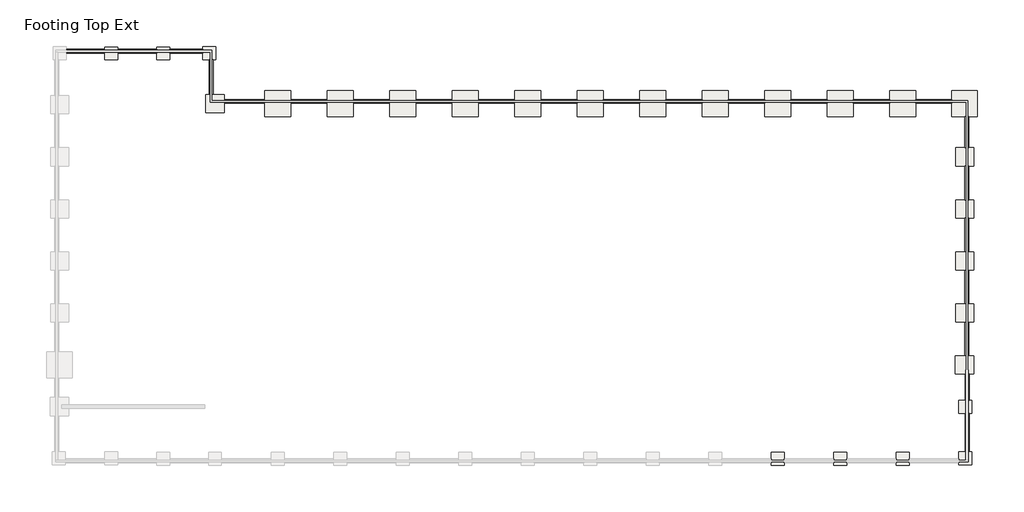
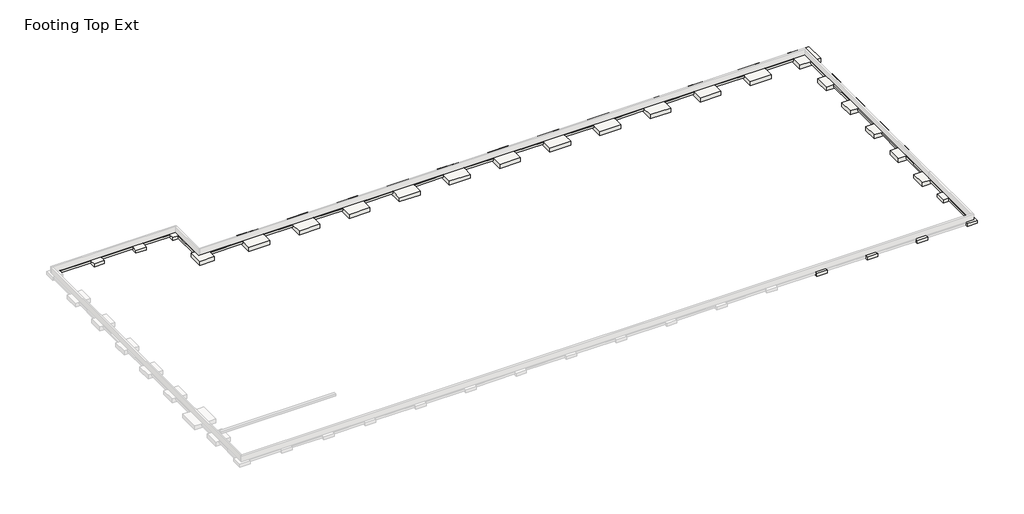
# One storey, part 2 of 2: 26 slabs, 5 footings.
"""IFC4 building model written with IfcOpenShell, lengths in millimetres."""

from ifc_helpers import new_model, si_unit, frame, origin, place, context, project, spatial, polyline, outline, extrude, faceted_brep, element, save

model = new_model("IFC4")

# Units and contexts
model_context = context("Model", 3, world=origin())
ifc_project = project(units=[si_unit("LENGTHUNIT", "METRE", prefix="MILLI")], contexts=[model_context])

# Site, building, storey
site = spatial("IfcSite", under=ifc_project)
building = spatial("IfcBuilding", under=site)
storey = spatial("IfcBuildingStorey", under=building, Name="Footing Top Ext", Elevation=-914.4)

# Footings
placement = place(None, origin())
element("IfcFooting", 1, ObjectType="Bearing Footing - 18\" x 12\"", at=placement, inside=storey, context=model_context, shape_type="SweptSolid", body=[
    extrude(outline(polyline([(305697.0398264, -530975.6413841), (305697.0398264, -530518.4413841), (310230.9398264, -530518.4413841), (310230.9398264, -530975.6413841), (305697.0398264, -530975.6413841)])), frame((0.0, 0.0, -1219.2), z_axis=(0.0, 0.0, 1.0), x_axis=(1.0, 0.0, 0.0)), (0.0, 0.0, 1.0), 304.8),
    extrude(outline(polyline([(317882.6898264, -530975.6413841), (317882.6898264, -530518.4413841), (321806.9898264, -530518.4413841), (321806.9898264, -530975.6413841), (317882.6898264, -530975.6413841)])), frame((0.0, 0.0, -1219.2), z_axis=(0.0, 0.0, 1.0), x_axis=(1.0, 0.0, 0.0)), (0.0, 0.0, 1.0), 304.8),
    extrude(outline(polyline([(316358.6898264, -530518.4413841), (316358.6898264, -530975.6413841), (311754.9398264, -530975.6413841), (311754.9398264, -530518.4413841), (316358.6898264, -530518.4413841)])), frame((0.0, 0.0, -1219.2), z_axis=(0.0, 0.0, 1.0), x_axis=(1.0, 0.0, 0.0)), (0.0, 0.0, 1.0), 304.8),
])
element("IfcFooting", 2, ObjectType="Bearing Footing - 18\" x 12\"", at=placement, inside=storey, context=model_context, shape_type="SweptSolid", body=[
    extrude(outline(polyline([(322537.2398264, -531712.2413841), (322994.4398264, -531712.2413841), (322994.4398264, -535839.7413841), (322537.2398264, -535839.7413841), (322537.2398264, -531712.2413841)])), frame((0.0, 0.0, -1219.2), z_axis=(0.0, 0.0, 1.0), x_axis=(1.0, 0.0, 0.0)), (0.0, 0.0, 1.0), 304.8),
])
element("IfcFooting", 3, ObjectType="Bearing Footing - 18\" x 12\"", at=placement, inside=storey, context=model_context, shape_type="SweptSolid", body=[
    extrude(outline(polyline([(409862.4397781, -536430.2913841), (409862.4397781, -536887.4913841), (405658.7398264, -536887.4913841), (405658.7398264, -536430.2913841), (409862.4397781, -536430.2913841)])), frame((0.0, 0.0, -1219.2), z_axis=(0.0, 0.0, 1.0), x_axis=(1.0, 0.0, 0.0)), (0.0, 0.0, 1.0), 304.8),
    extrude(outline(polyline([(402610.7398264, -536430.2913841), (402610.7398264, -536887.4913841), (398305.4398264, -536887.4913841), (398305.4398264, -536430.2913841), (402610.7398264, -536430.2913841)])), frame((0.0, 0.0, -1219.2), z_axis=(0.0, 0.0, 1.0), x_axis=(1.0, 0.0, 0.0)), (0.0, 0.0, 1.0), 304.8),
    extrude(outline(polyline([(395257.4398264, -536430.2913841), (395257.4398264, -536887.4913841), (390952.1398264, -536887.4913841), (390952.1398264, -536430.2913841), (395257.4398264, -536430.2913841)])), frame((0.0, 0.0, -1219.2), z_axis=(0.0, 0.0, 1.0), x_axis=(1.0, 0.0, 0.0)), (0.0, 0.0, 1.0), 304.8),
    extrude(outline(polyline([(387904.1398264, -536430.2913841), (387904.1398264, -536887.4913841), (383598.8398264, -536887.4913841), (383598.8398264, -536430.2913841), (387904.1398264, -536430.2913841)])), frame((0.0, 0.0, -1219.2), z_axis=(0.0, 0.0, 1.0), x_axis=(1.0, 0.0, 0.0)), (0.0, 0.0, 1.0), 304.8),
    extrude(outline(polyline([(380550.8398264, -536430.2913841), (380550.8398264, -536887.4913841), (376245.5398264, -536887.4913841), (376245.5398264, -536430.2913841), (380550.8398264, -536430.2913841)])), frame((0.0, 0.0, -1219.2), z_axis=(0.0, 0.0, 1.0), x_axis=(1.0, 0.0, 0.0)), (0.0, 0.0, 1.0), 304.8),
    extrude(outline(polyline([(373197.5398264, -536430.2913841), (373197.5398264, -536887.4913841), (368892.2398264, -536887.4913841), (368892.2398264, -536430.2913841), (373197.5398264, -536430.2913841)])), frame((0.0, 0.0, -1219.2), z_axis=(0.0, 0.0, 1.0), x_axis=(1.0, 0.0, 0.0)), (0.0, 0.0, 1.0), 304.8),
    extrude(outline(polyline([(365844.2398264, -536430.2913841), (365844.2398264, -536887.4913841), (361538.9398264, -536887.4913841), (361538.9398264, -536430.2913841), (365844.2398264, -536430.2913841)])), frame((0.0, 0.0, -1219.2), z_axis=(0.0, 0.0, 1.0), x_axis=(1.0, 0.0, 0.0)), (0.0, 0.0, 1.0), 304.8),
    extrude(outline(polyline([(358490.9398264, -536430.2913841), (358490.9398264, -536887.4913841), (354185.6398264, -536887.4913841), (354185.6398264, -536430.2913841), (358490.9398264, -536430.2913841)])), frame((0.0, 0.0, -1219.2), z_axis=(0.0, 0.0, 1.0), x_axis=(1.0, 0.0, 0.0)), (0.0, 0.0, 1.0), 304.8),
    extrude(outline(polyline([(351137.6398264, -536430.2913841), (351137.6398264, -536887.4913841), (346832.3398264, -536887.4913841), (346832.3398264, -536430.2913841), (351137.6398264, -536430.2913841)])), frame((0.0, 0.0, -1219.2), z_axis=(0.0, 0.0, 1.0), x_axis=(1.0, 0.0, 0.0)), (0.0, 0.0, 1.0), 304.8),
    extrude(outline(polyline([(343784.3398264, -536430.2913841), (343784.3398264, -536887.4913841), (339479.0398264, -536887.4913841), (339479.0398264, -536430.2913841), (343784.3398264, -536430.2913841)])), frame((0.0, 0.0, -1219.2), z_axis=(0.0, 0.0, 1.0), x_axis=(1.0, 0.0, 0.0)), (0.0, 0.0, 1.0), 304.8),
    extrude(outline(polyline([(336431.0398264, -536430.2913841), (336431.0398264, -536887.4913841), (332125.7398264, -536887.4913841), (332125.7398264, -536430.2913841), (336431.0398264, -536430.2913841)])), frame((0.0, 0.0, -1219.2), z_axis=(0.0, 0.0, 1.0), x_axis=(1.0, 0.0, 0.0)), (0.0, 0.0, 1.0), 304.8),
    extrude(outline(polyline([(329077.7398264, -536430.2913841), (329077.7398264, -536887.4913841), (324289.8398264, -536887.4913841), (324289.8398264, -536430.2913841), (329077.7398264, -536430.2913841)])), frame((0.0, 0.0, -1219.2), z_axis=(0.0, 0.0, 1.0), x_axis=(1.0, 0.0, 0.0)), (0.0, 0.0, 1.0), 304.8),
])
element("IfcFooting", 4, ObjectType="Bearing Footing - 18\" x 12\"", at=placement, inside=storey, context=model_context, shape_type="SweptSolid", body=[
    extrude(outline(polyline([(411894.4398264, -560496.7913841), (411437.2398264, -560496.7913841), (411437.2398264, -556502.6413841), (411894.4398264, -556502.6413841), (411894.4398264, -560496.7913841)])), frame((0.0, 0.0, -1219.2), z_axis=(0.0, 0.0, 1.0), x_axis=(1.0, 0.0, 0.0)), (0.0, 0.0, 1.0), 304.8),
    extrude(outline(polyline([(411437.2398264, -562630.3913841), (411894.4398264, -562630.3913841), (411894.4398264, -566599.1414082), (411437.2398264, -566599.1414082), (411437.2398264, -562630.3913841)])), frame((0.0, 0.0, -1219.2), z_axis=(0.0, 0.0, 1.0), x_axis=(1.0, 0.0, 0.0)), (0.0, 0.0, 1.0), 304.8),
    extrude(outline(polyline([(411894.4398264, -554369.0413841), (411437.2398264, -554369.0413841), (411437.2398264, -550374.8913841), (411894.4398264, -550374.8913841), (411894.4398264, -554369.0413841)])), frame((0.0, 0.0, -1219.2), z_axis=(0.0, 0.0, 1.0), x_axis=(1.0, 0.0, 0.0)), (0.0, 0.0, 1.0), 304.8),
    extrude(outline(polyline([(411894.4398264, -548241.2913841), (411437.2398264, -548241.2913841), (411437.2398264, -544247.1413841), (411894.4398264, -544247.1413841), (411894.4398264, -548241.2913841)])), frame((0.0, 0.0, -1219.2), z_axis=(0.0, 0.0, 1.0), x_axis=(1.0, 0.0, 0.0)), (0.0, 0.0, 1.0), 304.8),
    extrude(outline(polyline([(411894.4398264, -542113.5413841), (411437.2398264, -542113.5413841), (411437.2398264, -538424.1913358), (411894.4398264, -538424.1913358), (411894.4398264, -542113.5413841)])), frame((0.0, 0.0, -1219.2), z_axis=(0.0, 0.0, 1.0), x_axis=(1.0, 0.0, 0.0)), (0.0, 0.0, 1.0), 304.8),
])
element("IfcFooting", 5, ObjectType="Bearing Footing - 18\" x 12\"", at=placement, inside=storey, context=model_context, shape_type="SweptSolid", body=[
    extrude(outline(polyline([(411932.5398264, -571831.5413841), (411475.3398264, -571831.5413841), (411475.3398264, -568732.7414082), (411932.5398264, -568732.7414082), (411932.5398264, -571831.5413841)])), frame((0.0, 0.0, -1219.2), z_axis=(0.0, 0.0, 1.0), x_axis=(1.0, 0.0, 0.0)), (0.0, 0.0, 1.0), 304.8),
    extrude(outline(polyline([(411475.3398264, -573355.5413841), (411932.5398264, -573355.5413841), (411932.5398264, -577927.5413841), (411475.3398264, -577927.5413841), (411475.3398264, -573355.5413841)])), frame((0.0, 0.0, -1219.2), z_axis=(0.0, 0.0, 1.0), x_axis=(1.0, 0.0, 0.0)), (0.0, 0.0, 1.0), 304.8),
])

# Slabs
element("IfcSlab", 6, ObjectType="Footing-Rectangular : F10", at=placement, inside=storey, context=model_context, shape_type="Brep", body=[
    faceted_brep([(409862.4397781, -535376.1913358, -914.4), (409862.4397781, -536430.2913841, -914.4), (409862.4397781, -536887.4913841, -914.4), (409862.4397781, -538424.1913358, -914.4), (411437.2398264, -538424.1913358, -914.4), (411894.4398264, -538424.1913358, -914.4), (412910.4397781, -538424.1913358, -914.4), (412910.4397781, -535376.1913358, -914.4), (409862.4397781, -535376.1913358, -1524.0), (412910.4397781, -535376.1913358, -1524.0), (412910.4397781, -538424.1913358, -1524.0), (409862.4397781, -538424.1913358, -1524.0)], [[[0, 1, 2, 3, 4, 5, 6, 7]], [[8, 9, 10, 11]], [[3, 2, 1, 0, 8, 11]], [[6, 5, 4, 3, 11, 10]], [[7, 6, 10, 9]], [[0, 7, 9, 8]]]),
])
element("IfcSlab", 7, ObjectType="Footing-Rectangular : F10", at=placement, inside=storey, context=model_context, shape_type="Brep", body=[
    faceted_brep([(402610.7398264, -535382.5413358, -914.4), (402610.7398264, -536430.2913841, -914.4), (402610.7398264, -536887.4913841, -914.4), (402610.7398264, -538430.5413358, -914.4), (405658.7398264, -538430.5413358, -914.4), (405658.7398264, -536887.4913841, -914.4), (405658.7398264, -536430.2913841, -914.4), (405658.7398264, -535382.5413358, -914.4), (402610.7398264, -535382.5413358, -1524.0), (405658.7398264, -535382.5413358, -1524.0), (405658.7398264, -538430.5413358, -1524.0), (402610.7398264, -538430.5413358, -1524.0)], [[[0, 1, 2, 3, 4, 5, 6, 7]], [[8, 9, 10, 11]], [[3, 2, 1, 0, 8, 11]], [[4, 3, 11, 10]], [[7, 6, 5, 4, 10, 9]], [[0, 7, 9, 8]]]),
])
element("IfcSlab", 8, ObjectType="Footing-Rectangular : F10", at=placement, inside=storey, context=model_context, shape_type="Brep", body=[
    faceted_brep([(395257.4398264, -535382.5413358, -914.4), (395257.4398264, -536430.2913841, -914.4), (395257.4398264, -536887.4913841, -914.4), (395257.4398264, -538430.5413358, -914.4), (398305.4398264, -538430.5413358, -914.4), (398305.4398264, -536887.4913841, -914.4), (398305.4398264, -536430.2913841, -914.4), (398305.4398264, -535382.5413358, -914.4), (395257.4398264, -535382.5413358, -1524.0), (398305.4398264, -535382.5413358, -1524.0), (398305.4398264, -538430.5413358, -1524.0), (395257.4398264, -538430.5413358, -1524.0)], [[[0, 1, 2, 3, 4, 5, 6, 7]], [[8, 9, 10, 11]], [[3, 2, 1, 0, 8, 11]], [[4, 3, 11, 10]], [[7, 6, 5, 4, 10, 9]], [[0, 7, 9, 8]]]),
])
element("IfcSlab", 9, ObjectType="Footing-Rectangular : F10", at=placement, inside=storey, context=model_context, shape_type="Brep", body=[
    faceted_brep([(387904.1398264, -535382.5413358, -914.4), (387904.1398264, -536430.2913841, -914.4), (387904.1398264, -536887.4913841, -914.4), (387904.1398264, -538430.5413358, -914.4), (390952.1398264, -538430.5413358, -914.4), (390952.1398264, -536887.4913841, -914.4), (390952.1398264, -536430.2913841, -914.4), (390952.1398264, -535382.5413358, -914.4), (387904.1398264, -535382.5413358, -1524.0), (390952.1398264, -535382.5413358, -1524.0), (390952.1398264, -538430.5413358, -1524.0), (387904.1398264, -538430.5413358, -1524.0)], [[[0, 1, 2, 3, 4, 5, 6, 7]], [[8, 9, 10, 11]], [[3, 2, 1, 0, 8, 11]], [[4, 3, 11, 10]], [[7, 6, 5, 4, 10, 9]], [[0, 7, 9, 8]]]),
])
element("IfcSlab", 10, ObjectType="Footing-Rectangular : F10", at=placement, inside=storey, context=model_context, shape_type="Brep", body=[
    faceted_brep([(380550.8398264, -535382.5413358, -914.4), (380550.8398264, -536430.2913841, -914.4), (380550.8398264, -536887.4913841, -914.4), (380550.8398264, -538430.5413358, -914.4), (383598.8398264, -538430.5413358, -914.4), (383598.8398264, -536887.4913841, -914.4), (383598.8398264, -536430.2913841, -914.4), (383598.8398264, -535382.5413358, -914.4), (380550.8398264, -535382.5413358, -1524.0), (383598.8398264, -535382.5413358, -1524.0), (383598.8398264, -538430.5413358, -1524.0), (380550.8398264, -538430.5413358, -1524.0)], [[[0, 1, 2, 3, 4, 5, 6, 7]], [[8, 9, 10, 11]], [[3, 2, 1, 0, 8, 11]], [[4, 3, 11, 10]], [[7, 6, 5, 4, 10, 9]], [[0, 7, 9, 8]]]),
])
element("IfcSlab", 11, ObjectType="Footing-Rectangular : F10", at=placement, inside=storey, context=model_context, shape_type="Brep", body=[
    faceted_brep([(373197.5398264, -535382.5413358, -914.4), (373197.5398264, -536430.2913841, -914.4), (373197.5398264, -536887.4913841, -914.4), (373197.5398264, -538430.5413358, -914.4), (376245.5398264, -538430.5413358, -914.4), (376245.5398264, -536887.4913841, -914.4), (376245.5398264, -536430.2913841, -914.4), (376245.5398264, -535382.5413358, -914.4), (373197.5398264, -535382.5413358, -1524.0), (376245.5398264, -535382.5413358, -1524.0), (376245.5398264, -538430.5413358, -1524.0), (373197.5398264, -538430.5413358, -1524.0)], [[[0, 1, 2, 3, 4, 5, 6, 7]], [[8, 9, 10, 11]], [[3, 2, 1, 0, 8, 11]], [[4, 3, 11, 10]], [[7, 6, 5, 4, 10, 9]], [[0, 7, 9, 8]]]),
])
element("IfcSlab", 12, ObjectType="Footing-Rectangular : F10", at=placement, inside=storey, context=model_context, shape_type="Brep", body=[
    faceted_brep([(365844.2398264, -535382.5413358, -914.4), (365844.2398264, -536430.2913841, -914.4), (365844.2398264, -536887.4913841, -914.4), (365844.2398264, -538430.5413358, -914.4), (368892.2398264, -538430.5413358, -914.4), (368892.2398264, -536887.4913841, -914.4), (368892.2398264, -536430.2913841, -914.4), (368892.2398264, -535382.5413358, -914.4), (365844.2398264, -535382.5413358, -1524.0), (368892.2398264, -535382.5413358, -1524.0), (368892.2398264, -538430.5413358, -1524.0), (365844.2398264, -538430.5413358, -1524.0)], [[[0, 1, 2, 3, 4, 5, 6, 7]], [[8, 9, 10, 11]], [[3, 2, 1, 0, 8, 11]], [[4, 3, 11, 10]], [[7, 6, 5, 4, 10, 9]], [[0, 7, 9, 8]]]),
])
element("IfcSlab", 13, ObjectType="Footing-Rectangular : F10", at=placement, inside=storey, context=model_context, shape_type="Brep", body=[
    faceted_brep([(358490.9398264, -535382.5413358, -914.4), (358490.9398264, -536430.2913841, -914.4), (358490.9398264, -536887.4913841, -914.4), (358490.9398264, -538430.5413358, -914.4), (361538.9398264, -538430.5413358, -914.4), (361538.9398264, -536887.4913841, -914.4), (361538.9398264, -536430.2913841, -914.4), (361538.9398264, -535382.5413358, -914.4), (358490.9398264, -535382.5413358, -1524.0), (361538.9398264, -535382.5413358, -1524.0), (361538.9398264, -538430.5413358, -1524.0), (358490.9398264, -538430.5413358, -1524.0)], [[[0, 1, 2, 3, 4, 5, 6, 7]], [[8, 9, 10, 11]], [[3, 2, 1, 0, 8, 11]], [[4, 3, 11, 10]], [[7, 6, 5, 4, 10, 9]], [[0, 7, 9, 8]]]),
])
element("IfcSlab", 14, ObjectType="Footing-Rectangular : F10", at=placement, inside=storey, context=model_context, shape_type="Brep", body=[
    faceted_brep([(351137.6398264, -535382.5413358, -914.4), (351137.6398264, -536430.2913841, -914.4), (351137.6398264, -536887.4913841, -914.4), (351137.6398264, -538430.5413358, -914.4), (354185.6398264, -538430.5413358, -914.4), (354185.6398264, -536887.4913841, -914.4), (354185.6398264, -536430.2913841, -914.4), (354185.6398264, -535382.5413358, -914.4), (351137.6398264, -535382.5413358, -1524.0), (354185.6398264, -535382.5413358, -1524.0), (354185.6398264, -538430.5413358, -1524.0), (351137.6398264, -538430.5413358, -1524.0)], [[[0, 1, 2, 3, 4, 5, 6, 7]], [[8, 9, 10, 11]], [[3, 2, 1, 0, 8, 11]], [[4, 3, 11, 10]], [[7, 6, 5, 4, 10, 9]], [[0, 7, 9, 8]]]),
])
element("IfcSlab", 15, ObjectType="Footing-Rectangular : F10", at=placement, inside=storey, context=model_context, shape_type="Brep", body=[
    faceted_brep([(343784.3398264, -535382.5413358, -914.4), (343784.3398264, -536430.2913841, -914.4), (343784.3398264, -536887.4913841, -914.4), (343784.3398264, -538430.5413358, -914.4), (346832.3398264, -538430.5413358, -914.4), (346832.3398264, -536887.4913841, -914.4), (346832.3398264, -536430.2913841, -914.4), (346832.3398264, -535382.5413358, -914.4), (343784.3398264, -535382.5413358, -1524.0), (346832.3398264, -535382.5413358, -1524.0), (346832.3398264, -538430.5413358, -1524.0), (343784.3398264, -538430.5413358, -1524.0)], [[[0, 1, 2, 3, 4, 5, 6, 7]], [[8, 9, 10, 11]], [[3, 2, 1, 0, 8, 11]], [[4, 3, 11, 10]], [[7, 6, 5, 4, 10, 9]], [[0, 7, 9, 8]]]),
])
element("IfcSlab", 16, ObjectType="Footing-Rectangular : F10", at=placement, inside=storey, context=model_context, shape_type="Brep", body=[
    faceted_brep([(336431.0398264, -535382.5413358, -914.4), (336431.0398264, -536430.2913841, -914.4), (336431.0398264, -536887.4913841, -914.4), (336431.0398264, -538430.5413358, -914.4), (339479.0398264, -538430.5413358, -914.4), (339479.0398264, -536887.4913841, -914.4), (339479.0398264, -536430.2913841, -914.4), (339479.0398264, -535382.5413358, -914.4), (336431.0398264, -535382.5413358, -1524.0), (339479.0398264, -535382.5413358, -1524.0), (339479.0398264, -538430.5413358, -1524.0), (336431.0398264, -538430.5413358, -1524.0)], [[[0, 1, 2, 3, 4, 5, 6, 7]], [[8, 9, 10, 11]], [[3, 2, 1, 0, 8, 11]], [[4, 3, 11, 10]], [[7, 6, 5, 4, 10, 9]], [[0, 7, 9, 8]]]),
])
element("IfcSlab", 17, ObjectType="Footing-Rectangular : F10", at=placement, inside=storey, context=model_context, shape_type="Brep", body=[
    faceted_brep([(329077.7398264, -535382.5413358, -914.4), (329077.7398264, -536430.2913841, -914.4), (329077.7398264, -536887.4913841, -914.4), (329077.7398264, -538430.5413358, -914.4), (332125.7398264, -538430.5413358, -914.4), (332125.7398264, -536887.4913841, -914.4), (332125.7398264, -536430.2913841, -914.4), (332125.7398264, -535382.5413358, -914.4), (329077.7398264, -535382.5413358, -1524.0), (332125.7398264, -535382.5413358, -1524.0), (332125.7398264, -538430.5413358, -1524.0), (329077.7398264, -538430.5413358, -1524.0)], [[[0, 1, 2, 3, 4, 5, 6, 7]], [[8, 9, 10, 11]], [[3, 2, 1, 0, 8, 11]], [[4, 3, 11, 10]], [[7, 6, 5, 4, 10, 9]], [[0, 7, 9, 8]]]),
])
element("IfcSlab", 18, ObjectType="Footing-Rectangular : F5", at=placement, inside=storey, context=model_context, shape_type="Brep", body=[
    faceted_brep([(317882.6898264, -530245.3913841, -914.4), (316358.6898264, -530245.3913841, -914.4), (316358.6898264, -530518.4413841, -914.4), (316358.6898264, -530975.6413841, -914.4), (316358.6898264, -531769.3913841, -914.4), (317882.6898264, -531769.3913841, -914.4), (317882.6898264, -530975.6413841, -914.4), (317882.6898264, -530518.4413841, -914.4), (317882.6898264, -530245.3913841, -1371.6), (317882.6898264, -531769.3913841, -1371.6), (316358.6898264, -531769.3913841, -1371.6), (316358.6898264, -530245.3913841, -1371.6)], [[[0, 1, 2, 3, 4, 5, 6, 7]], [[8, 9, 10, 11]], [[1, 0, 8, 11]], [[4, 3, 2, 1, 11, 10]], [[5, 4, 10, 9]], [[0, 7, 6, 5, 9, 8]]]),
])
element("IfcSlab", 19, ObjectType="Footing-Rectangular : F5", at=placement, inside=storey, context=model_context, shape_type="Brep", body=[
    faceted_brep([(311754.9398264, -530245.3913841, -914.4), (310230.9398264, -530245.3913841, -914.4), (310230.9398264, -530518.4413841, -914.4), (310230.9398264, -530975.6413841, -914.4), (310230.9398264, -531769.3913841, -914.4), (311754.9398264, -531769.3913841, -914.4), (311754.9398264, -530975.6413841, -914.4), (311754.9398264, -530518.4413841, -914.4), (311754.9398264, -530245.3913841, -1371.6), (311754.9398264, -531769.3913841, -1371.6), (310230.9398264, -531769.3913841, -1371.6), (310230.9398264, -530245.3913841, -1371.6)], [[[0, 1, 2, 3, 4, 5, 6, 7]], [[8, 9, 10, 11]], [[1, 0, 8, 11]], [[4, 3, 2, 1, 11, 10]], [[5, 4, 10, 9]], [[0, 7, 6, 5, 9, 8]]]),
])
element("IfcSlab", 20, ObjectType="Footing-Rectangular : F5", at=placement, inside=storey, context=model_context, shape_type="Brep", body=[
    faceted_brep([(323330.9898264, -530188.2413841, -914.4), (321806.9898264, -530188.2413841, -914.4), (321806.9898264, -530518.4413841, -914.4), (321806.9898264, -530975.6413841, -914.4), (321806.9898264, -531712.2413841, -914.4), (322537.2398264, -531712.2413841, -914.4), (322994.4398264, -531712.2413841, -914.4), (323330.9898264, -531712.2413841, -914.4), (323330.9898264, -530188.2413841, -1371.6), (323330.9898264, -531712.2413841, -1371.6), (321806.9898264, -531712.2413841, -1371.6), (321806.9898264, -530188.2413841, -1371.6)], [[[0, 1, 2, 3, 4, 5, 6, 7]], [[8, 9, 10, 11]], [[1, 0, 8, 11]], [[4, 3, 2, 1, 11, 10]], [[7, 6, 5, 4, 10, 9]], [[0, 7, 9, 8]]]),
])
element("IfcSlab", 21, ObjectType="Footing-Rectangular : F5", at=placement, inside=storey, context=model_context, shape_type="Brep", body=[
    faceted_brep([(390190.1398264, -577978.3413841, -914.4), (388666.1398264, -577978.3413841, -914.4), (388666.1398264, -578759.3913841, -914.4), (388666.1398264, -579216.5913841, -914.4), (388666.1398264, -579502.3413841, -914.4), (390190.1398264, -579502.3413841, -914.4), (390190.1398264, -579216.5913841, -914.4), (390190.1398264, -578759.3913841, -914.4), (390190.1398264, -577978.3413841, -1371.6), (390190.1398264, -579502.3413841, -1371.6), (388666.1398264, -579502.3413841, -1371.6), (388666.1398264, -577978.3413841, -1371.6)], [[[0, 1, 2, 3, 4, 5, 6, 7]], [[8, 9, 10, 11]], [[1, 0, 8, 11]], [[4, 3, 2, 1, 11, 10]], [[5, 4, 10, 9]], [[0, 7, 6, 5, 9, 8]]]),
])
element("IfcSlab", 22, ObjectType="Footing-Rectangular : F5", at=placement, inside=storey, context=model_context, shape_type="Brep", body=[
    faceted_brep([(397543.4398264, -577971.9913841, -914.4), (396019.4398264, -577971.9913841, -914.4), (396019.4398264, -578759.3913841, -914.4), (396019.4398264, -579216.5913841, -914.4), (396019.4398264, -579495.9913841, -914.4), (397543.4398264, -579495.9913841, -914.4), (397543.4398264, -579216.5913841, -914.4), (397543.4398264, -578759.3913841, -914.4), (397543.4398264, -577971.9913841, -1371.6), (397543.4398264, -579495.9913841, -1371.6), (396019.4398264, -579495.9913841, -1371.6), (396019.4398264, -577971.9913841, -1371.6)], [[[0, 1, 2, 3, 4, 5, 6, 7]], [[8, 9, 10, 11]], [[1, 0, 8, 11]], [[4, 3, 2, 1, 11, 10]], [[5, 4, 10, 9]], [[0, 7, 6, 5, 9, 8]]]),
])
element("IfcSlab", 23, ObjectType="Footing-Rectangular : F5", at=placement, inside=storey, context=model_context, shape_type="Brep", body=[
    faceted_brep([(404896.7398264, -577971.9913841, -914.4), (403372.7398264, -577971.9913841, -914.4), (403372.7398264, -578759.3913841, -914.4), (403372.7398264, -579216.5913841, -914.4), (403372.7398264, -579495.9913841, -914.4), (404896.7398264, -579495.9913841, -914.4), (404896.7398264, -579216.5913841, -914.4), (404896.7398264, -578759.3913841, -914.4), (404896.7398264, -577971.9913841, -1371.6), (404896.7398264, -579495.9913841, -1371.6), (403372.7398264, -579495.9913841, -1371.6), (403372.7398264, -577971.9913841, -1371.6)], [[[0, 1, 2, 3, 4, 5, 6, 7]], [[8, 9, 10, 11]], [[1, 0, 8, 11]], [[4, 3, 2, 1, 11, 10]], [[5, 4, 10, 9]], [[0, 7, 6, 5, 9, 8]]]),
])
element("IfcSlab", 24, ObjectType="Footing-Rectangular : F5", at=placement, inside=storey, context=model_context, shape_type="Brep", body=[
    faceted_brep([(412218.2898264, -571831.5413841, -914.4), (411932.5398264, -571831.5413841, -914.4), (411475.3398264, -571831.5413841, -914.4), (410694.2898264, -571831.5413841, -914.4), (410694.2898264, -573355.5413841, -914.4), (411475.3398264, -573355.5413841, -914.4), (411932.5398264, -573355.5413841, -914.4), (412218.2898264, -573355.5413841, -914.4), (412218.2898264, -571831.5413841, -1371.6), (412218.2898264, -573355.5413841, -1371.6), (410694.2898264, -573355.5413841, -1371.6), (410694.2898264, -571831.5413841, -1371.6)], [[[0, 1, 2, 3, 4, 5, 6, 7]], [[8, 9, 10, 11]], [[3, 2, 1, 0, 8, 11]], [[4, 3, 11, 10]], [[7, 6, 5, 4, 10, 9]], [[0, 7, 9, 8]]]),
])
element("IfcSlab", 25, ObjectType="Footing-Rectangular : F5", at=placement, inside=storey, context=model_context, shape_type="Brep", body=[
    faceted_brep([(412224.6398264, -577927.5413841, -914.4), (411932.5398264, -577927.5413841, -914.4), (411475.3398264, -577927.5413841, -914.4), (410700.6398264, -577927.5413841, -914.4), (410700.6398264, -578759.3913841, -914.4), (410700.6398264, -579216.5913841, -914.4), (410700.6398264, -579451.5413841, -914.4), (412224.6398264, -579451.5413841, -914.4), (412224.6398264, -577927.5413841, -1371.6), (412224.6398264, -579451.5413841, -1371.6), (410700.6398264, -579451.5413841, -1371.6), (410700.6398264, -577927.5413841, -1371.6)], [[[0, 1, 2, 3, 4, 5, 6, 7]], [[8, 9, 10, 11]], [[3, 2, 1, 0, 8, 11]], [[6, 5, 4, 3, 11, 10]], [[7, 6, 10, 9]], [[0, 7, 9, 8]]]),
])
element("IfcSlab", 26, ObjectType="Footing-Rectangular : F7", at=placement, inside=storey, context=model_context, shape_type="Brep", body=[
    faceted_brep([(410319.6398264, -566599.1414082, -914.4), (410319.6398264, -568732.7414082, -914.4), (411475.3398264, -568732.7414082, -914.4), (411932.5398264, -568732.7414082, -914.4), (412453.2398264, -568732.7414082, -914.4), (412453.2398264, -566599.1414082, -914.4), (411894.4398264, -566599.1414082, -914.4), (411437.2398264, -566599.1414082, -914.4), (410319.6398264, -566599.1414082, -1524.0), (412453.2398264, -566599.1414082, -1524.0), (412453.2398264, -568732.7414082, -1524.0), (410319.6398264, -568732.7414082, -1524.0)], [[[0, 1, 2, 3, 4, 5, 6, 7]], [[8, 9, 10, 11]], [[1, 0, 8, 11]], [[4, 3, 2, 1, 11, 10]], [[5, 4, 10, 9]], [[0, 7, 6, 5, 9, 8]]]),
])
element("IfcSlab", 27, ObjectType="Footing-Rectangular : F7", at=placement, inside=storey, context=model_context, shape_type="Brep", body=[
    faceted_brep([(412484.9898264, -560496.7913841, -914.4), (411894.4398264, -560496.7913841, -914.4), (411437.2398264, -560496.7913841, -914.4), (410351.3898264, -560496.7913841, -914.4), (410351.3898264, -562630.3913841, -914.4), (411437.2398264, -562630.3913841, -914.4), (411894.4398264, -562630.3913841, -914.4), (412484.9898264, -562630.3913841, -914.4), (412484.9898264, -560496.7913841, -1524.0), (412484.9898264, -562630.3913841, -1524.0), (410351.3898264, -562630.3913841, -1524.0), (410351.3898264, -560496.7913841, -1524.0)], [[[0, 1, 2, 3, 4, 5, 6, 7]], [[8, 9, 10, 11]], [[3, 2, 1, 0, 8, 11]], [[4, 3, 11, 10]], [[7, 6, 5, 4, 10, 9]], [[0, 7, 9, 8]]]),
])
element("IfcSlab", 28, ObjectType="Footing-Rectangular : F7", at=placement, inside=storey, context=model_context, shape_type="Brep", body=[
    faceted_brep([(412484.9898264, -554369.0413841, -914.4), (411894.4398264, -554369.0413841, -914.4), (411437.2398264, -554369.0413841, -914.4), (410351.3898264, -554369.0413841, -914.4), (410351.3898264, -556502.6413841, -914.4), (411437.2398264, -556502.6413841, -914.4), (411894.4398264, -556502.6413841, -914.4), (412484.9898264, -556502.6413841, -914.4), (412484.9898264, -554369.0413841, -1524.0), (412484.9898264, -556502.6413841, -1524.0), (410351.3898264, -556502.6413841, -1524.0), (410351.3898264, -554369.0413841, -1524.0)], [[[0, 1, 2, 3, 4, 5, 6, 7]], [[8, 9, 10, 11]], [[3, 2, 1, 0, 8, 11]], [[4, 3, 11, 10]], [[7, 6, 5, 4, 10, 9]], [[0, 7, 9, 8]]]),
])
element("IfcSlab", 29, ObjectType="Footing-Rectangular : F7", at=placement, inside=storey, context=model_context, shape_type="Brep", body=[
    faceted_brep([(412484.9898264, -548241.2913841, -914.4), (411894.4398264, -548241.2913841, -914.4), (411437.2398264, -548241.2913841, -914.4), (410351.3898264, -548241.2913841, -914.4), (410351.3898264, -550374.8913841, -914.4), (411437.2398264, -550374.8913841, -914.4), (411894.4398264, -550374.8913841, -914.4), (412484.9898264, -550374.8913841, -914.4), (412484.9898264, -548241.2913841, -1524.0), (412484.9898264, -550374.8913841, -1524.0), (410351.3898264, -550374.8913841, -1524.0), (410351.3898264, -548241.2913841, -1524.0)], [[[0, 1, 2, 3, 4, 5, 6, 7]], [[8, 9, 10, 11]], [[3, 2, 1, 0, 8, 11]], [[4, 3, 11, 10]], [[7, 6, 5, 4, 10, 9]], [[0, 7, 9, 8]]]),
])
element("IfcSlab", 30, ObjectType="Footing-Rectangular : F7", at=placement, inside=storey, context=model_context, shape_type="Brep", body=[
    faceted_brep([(412478.6398264, -542113.5413841, -914.4), (411894.4398264, -542113.5413841, -914.4), (411437.2398264, -542113.5413841, -914.4), (410345.0398264, -542113.5413841, -914.4), (410345.0398264, -544247.1413841, -914.4), (411437.2398264, -544247.1413841, -914.4), (411894.4398264, -544247.1413841, -914.4), (412478.6398264, -544247.1413841, -914.4), (412478.6398264, -542113.5413841, -1524.0), (412478.6398264, -544247.1413841, -1524.0), (410345.0398264, -544247.1413841, -1524.0), (410345.0398264, -542113.5413841, -1524.0)], [[[0, 1, 2, 3, 4, 5, 6, 7]], [[8, 9, 10, 11]], [[3, 2, 1, 0, 8, 11]], [[4, 3, 11, 10]], [[7, 6, 5, 4, 10, 9]], [[0, 7, 9, 8]]]),
])
element("IfcSlab", 31, ObjectType="Footing-Rectangular : F7", at=placement, inside=storey, context=model_context, shape_type="Brep", body=[
    faceted_brep([(322156.2398264, -535839.7413841, -914.4), (322156.2398264, -537973.3413841, -914.4), (324289.8398264, -537973.3413841, -914.4), (324289.8398264, -536887.4913841, -914.4), (324289.8398264, -536430.2913841, -914.4), (324289.8398264, -535839.7413841, -914.4), (322994.4398264, -535839.7413841, -914.4), (322537.2398264, -535839.7413841, -914.4), (322156.2398264, -535839.7413841, -1524.0), (324289.8398264, -535839.7413841, -1524.0), (324289.8398264, -537973.3413841, -1524.0), (322156.2398264, -537973.3413841, -1524.0)], [[[0, 1, 2, 3, 4, 5, 6, 7]], [[8, 9, 10, 11]], [[1, 0, 8, 11]], [[2, 1, 11, 10]], [[5, 4, 3, 2, 10, 9]], [[0, 7, 6, 5, 9, 8]]]),
])

save(model, "model.ifc")

# Revit data of these elements
# Type "Bearing Footing - 18\" x 12\""
#   Assembly Code = "A1010110"
# Type "Footing-Rectangular : F10"
#   Assembly Code = "A1010100"
#   Width = 10' - 0"
#   Length = 10' - 0"
#   Thickness = 2' - 0"
#   Structural Material [instance default] = CONCRETE FOOTING - SEE STRUCT DWGS.
# Type "Footing-Rectangular : F5"
#   Assembly Code = "A1010100"
#   Width = 5' - 0"
#   Length = 5' - 0"
#   Thickness = 1' - 6"
#   Structural Material [instance default] = CONCRETE FOOTING - SEE STRUCT DWGS.
# Type "Footing-Rectangular : F7"
#   Assembly Code = "A1010100"
#   Width = 7' - 0"
#   Length = 7' - 0"
#   Thickness = 2' - 0"
#   Structural Material [instance default] = CONCRETE FOOTING - SEE STRUCT DWGS.
# Elements 1, 2, 3, 4, 5 (IfcFooting, "Bearing Footing - 18\" x 12\"")
#   Phase Created = New Construction
#   Materials on its faces: "CONCRETE FOOTING - SEE STRUCT DWGS."
# Elements 6, 7, 8, 9, 10, 11, 12, 13, 14, 15, 16, 17 (IfcSlab, "Footing-Rectangular : F10")
#   Comments = ""
#   Structural Material = CONCRETE FOOTING - SEE STRUCT DWGS.
#   Phase Created = New Construction
#   Materials on its faces: "CONCRETE FOOTING - SEE STRUCT DWGS."
# Elements 18, 19, 20, 21, 22, 23, 24, 25 (IfcSlab, "Footing-Rectangular : F5")
#   Comments = ""
#   Structural Material = CONCRETE FOOTING - SEE STRUCT DWGS.
#   Phase Created = New Construction
#   Materials on its faces: "CONCRETE FOOTING - SEE STRUCT DWGS."
# Elements 26, 27, 28, 29, 30, 31 (IfcSlab, "Footing-Rectangular : F7")
#   Comments = ""
#   Structural Material = CONCRETE FOOTING - SEE STRUCT DWGS.
#   Phase Created = New Construction
#   Materials on its faces: "CONCRETE FOOTING - SEE STRUCT DWGS."
# Materials
#   "CONCRETE FOOTING - SEE STRUCT DWGS.": class "Concrete", colour RGB 192 192 192, transparency 0, Description = "Cast-in-place concrete", Cost = 0
